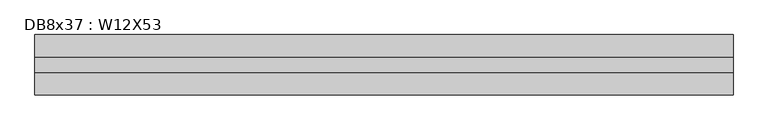
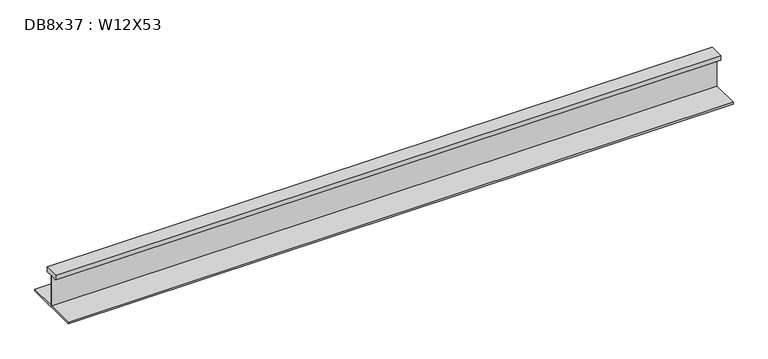
"""IFC4 building model written with IfcOpenShell, lengths in millimetres: beam geometry, DB8x37 : W12X53."""

from ifc_helpers import new_model, si_unit, frame, origin, place, context, project, spatial, polyline, outline, extrude, source, transform, mapped, element, save


def db8x37_w12x53_4f632cbe(model_context):
    return source(origin(), model_context, "Body", "SweptSolid", [
        extrude(outline(polyline([(38.1, 145.415), (38.1, 120.015), (2.921, 120.015), (2.921, -48.4505), (152.4, -48.4505), (152.4, -58.1025), (-152.4, -58.1025), (-152.4, -48.4505), (-2.921, -48.4505), (-2.921, 120.015), (-38.1, 120.015), (-38.1, 145.415), (38.1, 145.415)])), frame((-1760.9030956, 0.0, 0.0), z_axis=(1.0, 0.0, 0.0), x_axis=(0.0, 1.0, 0.0)), (0.0, 0.0, 1.0), 3528.892742),
    ])


if __name__ == "__main__":
    model = new_model("IFC4")
    model_context = context("Model", 3, world=origin())
    ifc_project = project(units=[si_unit("LENGTHUNIT", "METRE", prefix="MILLI")], contexts=[model_context])
    site = spatial("IfcSite", under=ifc_project)
    building = spatial("IfcBuilding", under=site)
    placement = place(None, origin())
    db8x37_w12x53_shape = db8x37_w12x53_4f632cbe(model_context)
    element("IfcBeam", 1, ObjectType="DB8x37 : W12X53", at=placement, inside=building, context=model_context, shape_type="MappedRepresentation", body=[
        mapped(db8x37_w12x53_shape, transform((0.0, 0.0, 0.0), x_axis=(1.0, 0.0, 0.0), y_axis=(0.0, 1.0, 0.0), z_axis=(0.0, 0.0, 1.0))),
    ])
    save(model, "model.ifc")

# Revit data of these elements
# Type "DB8x37 : W12X53"
#   Assembly Code = "B10"
#   W = 53
#   Length [instance default] = 5' - 0"
#   bf = 0' - 10"
#   d = 1' - 0.1"
#   k = 0' - 1 3/8"
#   k2 = 0' - 0.8"
#   tf = 0' - 0.575"
#   tw = 0' - 0.345"
#   A = 0.108333 SF
#   Structural Material [instance default] = Steel ASTM A992
# Element 1 (IfcBeam, "DB8x37 : W12X53")
#   Materials on its faces: "Steel ASTM A992"
# Materials
#   "Steel ASTM A992": class "Metal", colour RGB 199 199 199, transparency 0, Description = "Structural steel 50ksi", Cost = 0
